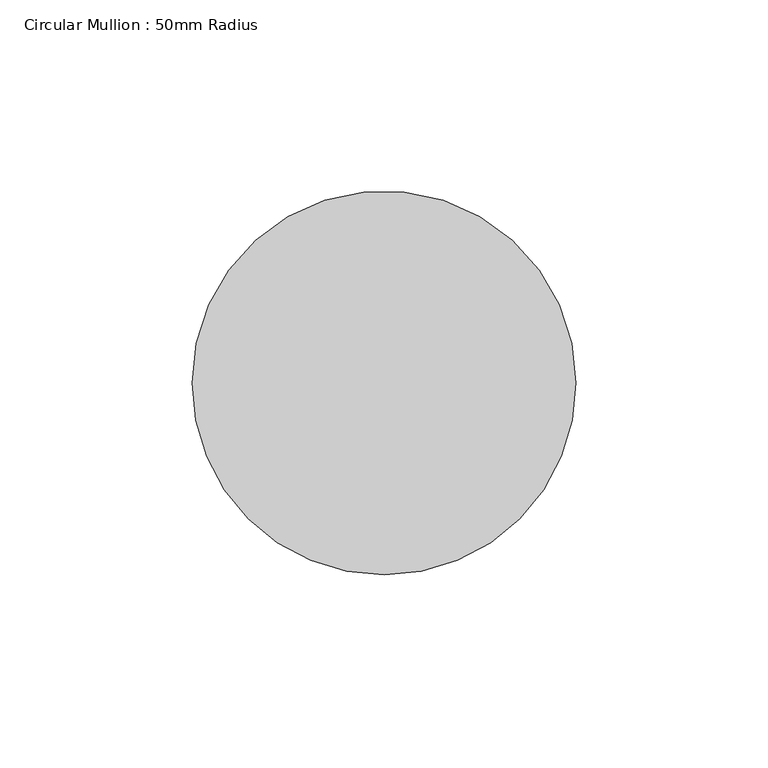
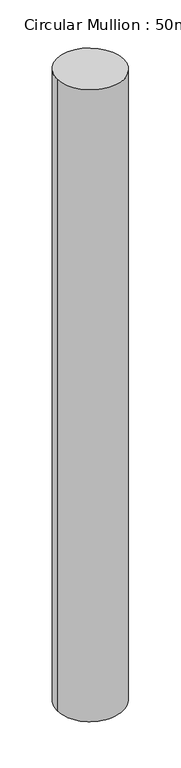
"""IFC4 building model written with IfcOpenShell, lengths in millimetres: member geometry, Circular Mullion : 50mm Radius."""

from ifc_helpers import new_model, si_unit, frame, origin, place, context, project, spatial, ellipse_curve, source, transform, mapped, element, save
from ifc_brep_helpers import plane_surface, cylinder_surface, advanced_brep


def circular_mullion_50mm_radius_1c708976(model_context):
    return source(origin(), model_context, "Body", "AdvancedBrep", [
        advanced_brep(
        [(-100.0, 0.0, 2.2947425), (0.0, 0.0, 0.0), (0.0, 0.0, -1003.5557998), (-100.0, 0.0, -1005.8405264)],
        [
            (0, 1, ellipse_curve(frame((-50.0, 0.0, 1.1473713), z_axis=(-0.022935777814390986, -0.022109758921082197, -0.9994924255123201), x_axis=(-0.7195868295624237, -0.6936713222966625, 0.03185735933028852)), 50.0253916, 50.0)),
            (1, 2),
            (2, 3, ellipse_curve(frame((-50.0, 0.0, -1004.6981631), z_axis=(-0.0228357699732062, -0.02201335280498372, 0.9994968433707103), x_axis=(0.7195900102095305, 0.6936743883946285, 0.031718450340230936)), 50.0251705, 50.0)),
            (3, 0),
            (1, 0, ellipse_curve(frame((-50.0, 0.0, 1.1473713), z_axis=(-0.022935777814390986, -0.022109758921082197, -0.9994924255123201), x_axis=(-0.7195868295624237, -0.6936713222966625, 0.03185735933028852)), 50.0253916, 50.0)),
            (3, 2, ellipse_curve(frame((-50.0, 0.0, -1004.6981631), z_axis=(-0.0228357699732062, -0.02201335280498372, 0.9994968433707103), x_axis=(0.7195900102095305, 0.6936743883946285, 0.031718450340230936)), 50.0251705, 50.0)),
        ],
        [
            cylinder_surface(frame((-50.0, 0.0, 0.0), z_axis=(0.0, 0.0, 1.0), x_axis=(1.0, 0.0, 0.0)), 50.0),
            plane_surface(frame((-211.5383905, 219.4414485, 0.0), z_axis=(0.022935777814390986, 0.022109758921082197, 0.9994924255123201), x_axis=(0.7195868295624237, 0.6936713222966624, -0.03185735933029421))),
            plane_surface(frame((-211.5383905, 219.4414485, -1003.5557998), z_axis=(0.0228357699732062, 0.02201335280498372, -0.9994968433707103), x_axis=(0.7195900102095305, 0.6936743883946285, 0.031718450340233684))),
        ],
        [
            (0, [[1, 2, 3, 4]]),
            (0, [[5, -4, 6, -2]]),
            (1, [[-1, -5]]),
            (2, [[-6, -3]]),
        ],
    ),
    ])


if __name__ == "__main__":
    model = new_model("IFC4")
    model_context = context("Model", 3, world=origin())
    ifc_project = project(units=[si_unit("LENGTHUNIT", "METRE", prefix="MILLI")], contexts=[model_context])
    site = spatial("IfcSite", under=ifc_project)
    building = spatial("IfcBuilding", under=site)
    placement = place(None, origin())
    circular_mullion_50mm_radius_shape = circular_mullion_50mm_radius_1c708976(model_context)
    element("IfcMember", 1, ObjectType="Circular Mullion : 50mm Radius", at=placement, inside=building, context=model_context, shape_type="MappedRepresentation", body=[
        mapped(circular_mullion_50mm_radius_shape, transform((0.0, 0.0, 0.0), x_axis=(1.0, 0.0, 0.0), y_axis=(0.0, 1.0, 0.0), z_axis=(0.0, 0.0, 1.0))),
    ])
    save(model, "model.ifc")

# Revit data of these elements
# Type "Circular Mullion : 50mm Radius"
#   built-in parameter 1007350 = 0.164042 (stored number, unit not read)
# Element 1 (IfcMember, "Circular Mullion : 50mm Radius")
#   Materials on its faces: "Aluminium"
# Materials
#   "Aluminium": class "Metal", colour RGB 247 247 247, transparency 0, Description = "Aluminium 6061", Cost = 0
